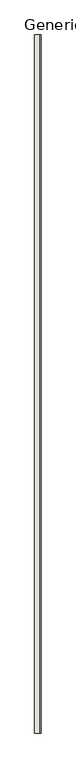
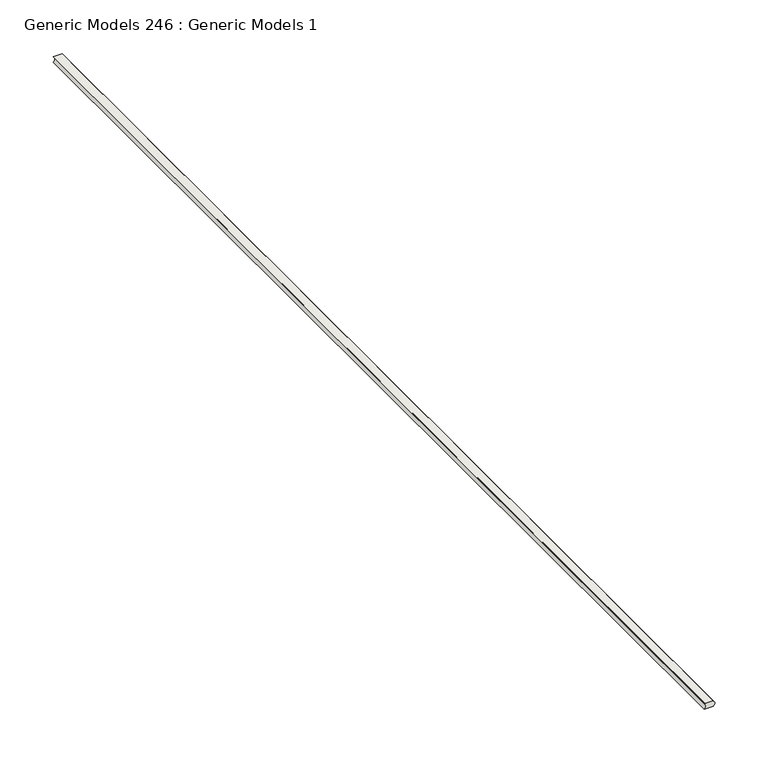
"""IFC4 building model written with IfcOpenShell, lengths in millimetres: wall geometry, Generic Models 246 : Generic Models 1."""

from ifc_helpers import new_model, si_unit, point, frame, frame_2d, origin, place, context, project, spatial, polyline, circle_curve, trimmed, segment, composite_curve, outline, extrude, source, transform, mapped, element, save


def generic_models_246_generic_models_1_38469833(model_context):
    return source(origin(), model_context, "Body", "SweptSolid", [
        extrude(outline(composite_curve([segment(polyline([(3048.0, 49679.225), (3048.0, 49688.75)]), True, "CONTINUOUS"), segment(trimmed(circle_curve(frame_2d((3051.175, 49685.8352595)), 4.3100275), [point((3048.0, 49688.75))], [point((3054.35, 49688.75))], False, "CARTESIAN"), True, "CONTINUOUS"), segment(polyline([(3054.35, 49688.75), (3054.35, 49679.225)]), True, "CONTINUOUS"), segment(trimmed(circle_curve(frame_2d((3051.175, 49676.3102595)), 4.3100275), [point((3054.35, 49679.225))], [point((3048.0, 49679.225))], True, "CARTESIAN"), True, "CONTINUOUS")], self_intersect=False)), frame((0.0, 0.0, 0.0), z_axis=(0.0, 1.0, 0.0), x_axis=(0.0, 0.0, 1.0)), (0.0, 0.0, 1.0), 1219.2),
    ])


if __name__ == "__main__":
    model = new_model("IFC4")
    model_context = context("Model", 3, world=origin())
    ifc_project = project(units=[si_unit("LENGTHUNIT", "METRE", prefix="MILLI")], contexts=[model_context])
    site = spatial("IfcSite", under=ifc_project)
    building = spatial("IfcBuilding", under=site)
    placement = place(None, origin())
    generic_models_246_generic_models_1_shape = generic_models_246_generic_models_1_38469833(model_context)
    element("IfcWall", 1, ObjectType="Generic Models 246 : Generic Models 1", at=placement, inside=building, context=model_context, shape_type="MappedRepresentation", body=[
        mapped(generic_models_246_generic_models_1_shape, transform((0.0, 0.0, 0.0), x_axis=(1.0, 0.0, 0.0), y_axis=(0.0, 1.0, 0.0), z_axis=(0.0, 0.0, 1.0))),
    ])
    save(model, "model.ifc")

# Revit data of these elements
# Element 1 (IfcWall, "Generic Models 246 : Generic Models 1")
#   Materials on its faces: "ACOUSTICAL SEALANT"
# Materials
#   "ACOUSTICAL SEALANT": class "Unassigned", colour RGB 120 120 120, transparency 0, Cost = 0
